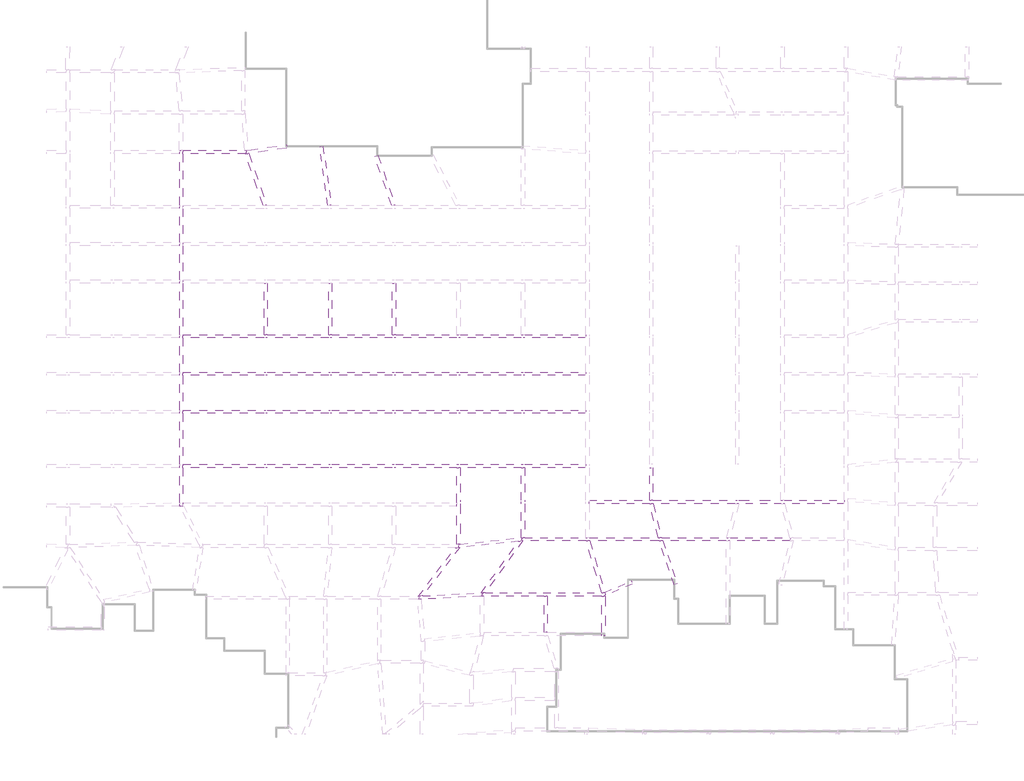
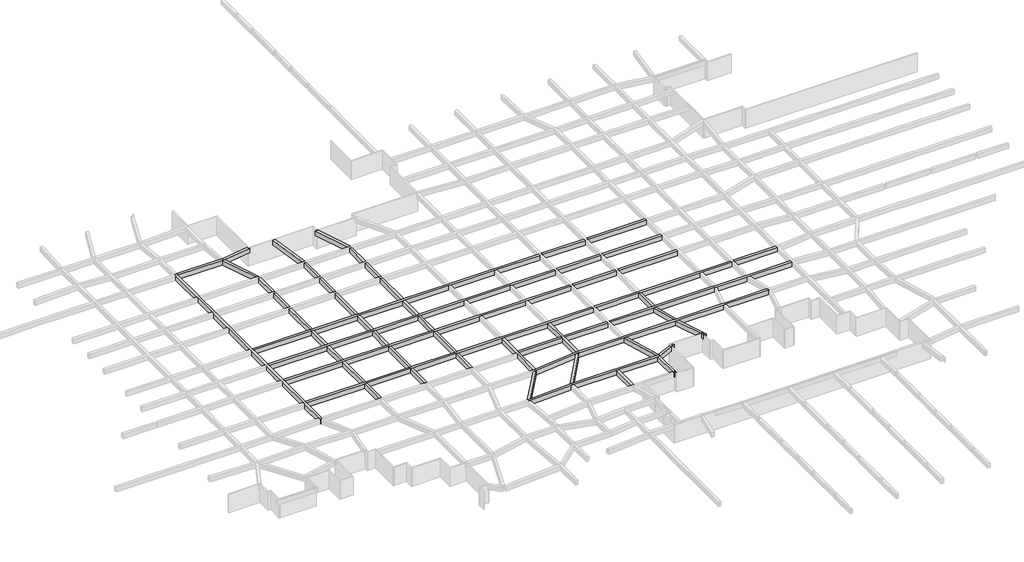
# One storey, part 33 of 45: 29 beams.
"""IFC4 building model written with IfcOpenShell, lengths in millimetres."""

from ifc_helpers import new_model, si_unit, frame, origin, place, context, project, spatial, polyline, outline, extrude, faceted_brep, element, save

model = new_model("IFC4")

# Units and contexts
model_context = context("Model", 3, world=origin())
ifc_project = project(units=[si_unit("LENGTHUNIT", "METRE", prefix="MILLI")], contexts=[model_context])

# Site, building, storey
site = spatial("IfcSite", under=ifc_project)
building = spatial("IfcBuilding", under=site)
storey = spatial("IfcBuildingStorey", under=building, Name="户型图", Elevation=0.0)

# Beams
placement = place(None, origin())
element("IfcBeam", 1, ObjectType="混凝土 - 矩形梁 : KL_beam", at=placement, inside=storey, context=model_context, shape_type="Brep", body=[
    faceted_brep([(-62329.0040152, 126289.9393475, 3300.0), (-62333.0898312, 126289.9393475, 3300.0), (-62729.0040152, 126289.9393475, 3300.0), (-62729.0040152, 125889.9393475, 3300.0), (-62729.0040152, 119677.6221749, 3300.0), (-62729.0040152, 119277.6221749, 3300.0), (-62729.0040152, 115171.853595, 3300.0), (-62729.0040152, 114771.853595, 3300.0), (-62729.0040152, 110629.932653, 3300.0), (-62729.0040152, 110229.932653, 3300.0), (-62729.0040152, 104011.2459144, 3300.0), (-62729.0040152, 103611.2459144, 3300.0), (-62729.0040152, 99488.7126183, 3300.0), (-62729.0040152, 99088.7126183, 3300.0), (-62729.0040152, 94888.7126183, 3300.0), (-62729.0040152, 94488.7126183, 3300.0), (-62729.0040152, 88347.4925836, 3300.0), (-62729.0040152, 87947.4925836, 3300.0), (-62729.0040152, 83686.8868717, 3300.0), (-62729.0040152, 83286.8331799, 3300.0), (-62652.5301432, 83288.0862256, 3300.0), (-62527.3655972, 83290.1370817, 3300.0), (-62329.0040152, 83293.3872917, 3300.0), (-62329.0040152, 83690.1370817, 3300.0), (-62329.0040152, 87947.4925836, 3300.0), (-62329.0040152, 88347.4925836, 3300.0), (-62329.0040152, 94488.7126183, 3300.0), (-62329.0040152, 94888.7126183, 3300.0), (-62329.0040152, 99088.7126183, 3300.0), (-62329.0040152, 99488.7126183, 3300.0), (-62329.0040152, 103611.2459144, 3300.0), (-62329.0040152, 104011.2459144, 3300.0), (-62329.0040152, 110229.932653, 3300.0), (-62329.0040152, 110629.932653, 3300.0), (-62329.0040152, 114771.853595, 3300.0), (-62329.0040152, 115171.853595, 3300.0), (-62329.0040152, 119262.5591329, 3300.0), (-62329.0040152, 119662.5591329, 3300.0), (-62329.0040152, 125890.334816, 3300.0), (-62729.0040152, 126289.9393475, 2500.0), (-62729.0040152, 125889.9393475, 2500.0), (-62729.0040152, 119677.6221749, 2500.0), (-62729.0040152, 119277.6221749, 2500.0), (-62729.0040152, 115171.853595, 2500.0), (-62729.0040152, 114771.853595, 2500.0), (-62729.0040152, 110629.932653, 2500.0), (-62729.0040152, 110229.932653, 2500.0), (-62729.0040152, 104011.2459144, 2500.0), (-62729.0040152, 103611.2459144, 2500.0), (-62729.0040152, 99488.7126183, 2500.0), (-62729.0040152, 99088.7126183, 2500.0), (-62729.0040152, 94888.7126183, 2500.0), (-62729.0040152, 94488.7126183, 2500.0), (-62729.0040152, 88347.4925836, 2500.0), (-62729.0040152, 87947.4925836, 2500.0), (-62729.0040152, 83686.8868717, 2500.0), (-62729.0040152, 83286.8331799, 2500.0), (-62333.0898312, 126289.9393475, 2500.0), (-62329.0040152, 126289.9393475, 2500.0), (-62329.0040152, 125890.334816, 2500.0), (-62329.0040152, 119662.5591329, 2500.0), (-62329.0040152, 119262.5591329, 2500.0), (-62329.0040152, 115171.853595, 2500.0), (-62329.0040152, 114771.853595, 2500.0), (-62329.0040152, 110629.932653, 2500.0), (-62329.0040152, 110229.932653, 2500.0), (-62329.0040152, 104011.2459144, 2500.0), (-62329.0040152, 103611.2459144, 2500.0), (-62329.0040152, 99488.7126183, 2500.0), (-62329.0040152, 99088.7126183, 2500.0), (-62329.0040152, 94888.7126183, 2500.0), (-62329.0040152, 94488.7126183, 2500.0), (-62329.0040152, 88347.4925836, 2500.0), (-62329.0040152, 87947.4925836, 2500.0), (-62329.0040152, 83690.1370817, 2500.0), (-62329.0040152, 83293.3872917, 2500.0), (-62527.3655972, 83290.1370817, 2500.0), (-62652.5301432, 83288.0862256, 2500.0)], [[[0, 1, 2, 3, 4, 5, 6, 7, 8, 9, 10, 11, 12, 13, 14, 15, 16, 17, 18, 19, 20, 21, 22, 23, 24, 25, 26, 27, 28, 29, 30, 31, 32, 33, 34, 35, 36, 37, 38]], [[2, 39, 40, 41, 42, 43, 44, 45, 46, 47, 48, 49, 50, 51, 52, 53, 54, 55, 56, 19, 18, 17, 16, 15, 14, 13, 12, 11, 10, 9, 8, 7, 6, 5, 4, 3]], [[39, 57, 58, 59, 60, 61, 62, 63, 64, 65, 66, 67, 68, 69, 70, 71, 72, 73, 74, 75, 76, 77, 56, 55, 54, 53, 52, 51, 50, 49, 48, 47, 46, 45, 44, 43, 42, 41, 40]], [[58, 0, 38, 37, 36, 35, 34, 33, 32, 31, 30, 29, 28, 27, 26, 25, 24, 23, 22, 75, 74, 73, 72, 71, 70, 69, 68, 67, 66, 65, 64, 63, 62, 61, 60, 59]], [[2, 1, 0, 58, 57, 39]], [[22, 21, 20, 19, 56, 77, 76, 75]]]),
])
element("IfcBeam", 2, ObjectType="混凝土 - 矩形梁 : KL_beam", at=placement, inside=storey, context=model_context, shape_type="Brep", body=[
    faceted_brep([(-62329.0040152, 125890.334816, 3300.0), (-54774.8544543, 125890.334816, 3300.0), (-54619.1044688, 125890.334816, 3300.0), (-54647.0751936, 126290.334816, 3300.0), (-54849.9735336, 126290.334816, 3300.0), (-62333.0898312, 126290.334816, 3300.0), (-62333.0898312, 126289.9393475, 3300.0), (-62329.0040152, 126289.9393475, 3300.0), (-62329.0040152, 125890.334816, 2500.0), (-54774.8544543, 125890.334816, 2500.0), (-54619.1044688, 125890.334816, 2500.0), (-62329.0040152, 126289.9393475, 2500.0), (-62333.0898312, 126289.9393475, 2500.0), (-62333.0898312, 126290.334816, 2500.0), (-54849.9735336, 126290.334816, 2500.0), (-54647.0751936, 126290.334816, 2500.0)], [[[0, 1, 2, 3, 4, 5, 6, 7]], [[2, 1, 0, 8, 9, 10]], [[10, 9, 8, 11, 12, 13, 14, 15]], [[3, 15, 14, 13, 5, 4]], [[7, 11, 8, 0]], [[11, 7, 6, 12]], [[6, 5, 13, 12]], [[3, 2, 10, 15]]]),
])
element("IfcBeam", 3, ObjectType="混凝土 - 矩形梁 : KL_beam", at=placement, inside=storey, context=model_context, shape_type="Brep", body=[
    faceted_brep([(-49808.6109146, 126970.3366244, 3300.0), (-49752.9416742, 126574.2293969, 3300.0), (-49752.9416742, 126574.2293969, 2500.0), (-49808.6109146, 126970.3366244, 2500.0), (-54450.8961138, 126317.9059876, 3300.0), (-54647.0751936, 126290.334816, 3300.0), (-54619.1044688, 125890.334816, 3300.0), (-54363.5430901, 125926.2516255, 3300.0), (-54619.1044688, 125890.334816, 2500.0), (-54363.5430901, 125926.2516255, 2500.0), (-54647.0751936, 126290.334816, 2500.0), (-54450.8961138, 126317.9059876, 2500.0)], [[[0, 1, 2, 3]], [[1, 0, 4, 5, 6, 7]], [[2, 1, 7, 6, 8, 9]], [[3, 2, 9, 8, 10, 11]], [[0, 3, 11, 10, 5, 4]], [[5, 10, 8, 6]]]),
])
element("IfcBeam", 4, ObjectType="混凝土 - 矩形梁 : KL_beam", at=placement, inside=storey, context=model_context, shape_type="Brep", body=[
    faceted_brep([(-62329.0040152, 104011.2459144, 3300.0), (-62329.0040152, 103611.2459144, 3300.0), (-52507.1090692, 103611.2459144, 3300.0), (-52107.1090692, 103611.2459144, 3300.0), (-44707.1090692, 103611.2459144, 3300.0), (-44307.1090692, 103611.2459144, 3300.0), (-36987.1090692, 103611.2459144, 3300.0), (-36587.1090692, 103611.2459144, 3300.0), (-29187.1090692, 103611.2459144, 3300.0), (-28787.1090692, 103611.2459144, 3300.0), (-21387.1090692, 103611.2459144, 3300.0), (-20987.1090692, 103611.2459144, 3300.0), (-13620.6748317, 103611.2459144, 3300.0), (-13620.6748317, 104011.2459144, 3300.0), (-20987.1090692, 104011.2459144, 3300.0), (-21387.1090692, 104011.2459144, 3300.0), (-28787.1090692, 104011.2459144, 3300.0), (-29187.1090692, 104011.2459144, 3300.0), (-36587.1090692, 104011.2459144, 3300.0), (-36987.1090692, 104011.2459144, 3300.0), (-44307.1090692, 104011.2459144, 3300.0), (-44707.1090692, 104011.2459144, 3300.0), (-52107.1090692, 104011.2459144, 3300.0), (-52507.1090692, 104011.2459144, 3300.0), (-62329.0040152, 103611.2459144, 2500.0), (-52507.1090692, 103611.2459144, 2500.0), (-52107.1090692, 103611.2459144, 2500.0), (-44707.1090692, 103611.2459144, 2500.0), (-44307.1090692, 103611.2459144, 2500.0), (-36987.1090692, 103611.2459144, 2500.0), (-36587.1090692, 103611.2459144, 2500.0), (-29187.1090692, 103611.2459144, 2500.0), (-28787.1090692, 103611.2459144, 2500.0), (-21387.1090692, 103611.2459144, 2500.0), (-20987.1090692, 103611.2459144, 2500.0), (-13620.6748317, 103611.2459144, 2500.0), (-62329.0040152, 104011.2459144, 2500.0), (-52507.1090692, 104011.2459144, 2500.0), (-52107.1090692, 104011.2459144, 2500.0), (-44707.1090692, 104011.2459144, 2500.0), (-44307.1090692, 104011.2459144, 2500.0), (-36987.1090692, 104011.2459144, 2500.0), (-36587.1090692, 104011.2459144, 2500.0), (-29187.1090692, 104011.2459144, 2500.0), (-28787.1090692, 104011.2459144, 2500.0), (-21387.1090692, 104011.2459144, 2500.0), (-20987.1090692, 104011.2459144, 2500.0), (-13620.6748317, 104011.2459144, 2500.0)], [[[0, 1, 2, 3, 4, 5, 6, 7, 8, 9, 10, 11, 12, 13, 14, 15, 16, 17, 18, 19, 20, 21, 22, 23]], [[1, 24, 25, 26, 27, 28, 29, 30, 31, 32, 33, 34, 35, 12, 11, 10, 9, 8, 7, 6, 5, 4, 3, 2]], [[24, 36, 37, 38, 39, 40, 41, 42, 43, 44, 45, 46, 47, 35, 34, 33, 32, 31, 30, 29, 28, 27, 26, 25]], [[36, 0, 23, 22, 21, 20, 19, 18, 17, 16, 15, 14, 13, 47, 46, 45, 44, 43, 42, 41, 40, 39, 38, 37]], [[1, 0, 36, 24]], [[13, 12, 35, 47]]]),
    faceted_brep([(-13220.6748317, 103611.2459144, 3300.0), (-13220.6748317, 104011.2459144, 3300.0), (-13220.6748317, 104011.2459144, 2500.0), (-13220.6748317, 103611.2459144, 2500.0), (-5904.3123934, 104011.2459144, 3300.0), (-5904.3123934, 103611.2459144, 3300.0), (-5904.3123934, 103611.2459144, 2500.0), (-5904.3123934, 104011.2459144, 2500.0)], [[[0, 1, 2, 3]], [[4, 5, 6, 7]], [[1, 0, 5, 4]], [[0, 3, 6, 5]], [[3, 2, 7, 6]], [[2, 1, 4, 7]]]),
    faceted_brep([(-5504.3123934, 104011.2459144, 3300.0), (-5504.3123934, 103611.2459144, 3300.0), (4500.9990644, 103611.2459144, 3300.0), (4500.9990644, 104011.2459144, 3300.0), (-5504.3123934, 103611.2459144, 2500.0), (4500.9990644, 103611.2459144, 2500.0), (-5504.3123934, 104011.2459144, 2500.0), (4500.9990644, 104011.2459144, 2500.0)], [[[0, 1, 2, 3]], [[1, 4, 5, 2]], [[4, 6, 7, 5]], [[6, 0, 3, 7]], [[1, 0, 6, 4]], [[3, 2, 5, 7]]]),
])
element("IfcBeam", 5, ObjectType="混凝土 - 矩形梁 : KL_beam", at=placement, inside=storey, context=model_context, shape_type="Brep", body=[
    faceted_brep([(-62329.0040152, 99488.7126183, 3300.0), (-62329.0040152, 99088.7126183, 3300.0), (-52507.1090692, 99088.7126183, 3300.0), (-52107.1090692, 99088.7126183, 3300.0), (-44707.1090692, 99088.7126183, 3300.0), (-44307.1090692, 99088.7126183, 3300.0), (-36987.1090692, 99088.7126183, 3300.0), (-36587.1090692, 99088.7126183, 3300.0), (-29187.1090692, 99088.7126183, 3300.0), (-28787.1090692, 99088.7126183, 3300.0), (-21387.1090692, 99088.7126183, 3300.0), (-20987.1090692, 99088.7126183, 3300.0), (-13620.6748317, 99088.7126183, 3300.0), (-13620.6748317, 99488.7126183, 3300.0), (-20987.1090692, 99488.7126183, 3300.0), (-21387.1090692, 99488.7126183, 3300.0), (-28787.1090692, 99488.7126183, 3300.0), (-29187.1090692, 99488.7126183, 3300.0), (-36587.1090692, 99488.7126183, 3300.0), (-36987.1090692, 99488.7126183, 3300.0), (-44307.1090692, 99488.7126183, 3300.0), (-44707.1090692, 99488.7126183, 3300.0), (-52107.1090692, 99488.7126183, 3300.0), (-52507.1090692, 99488.7126183, 3300.0), (-62329.0040152, 99088.7126183, 2500.0), (-52507.1090692, 99088.7126183, 2500.0), (-52107.1090692, 99088.7126183, 2500.0), (-44707.1090692, 99088.7126183, 2500.0), (-44307.1090692, 99088.7126183, 2500.0), (-36987.1090692, 99088.7126183, 2500.0), (-36587.1090692, 99088.7126183, 2500.0), (-29187.1090692, 99088.7126183, 2500.0), (-28787.1090692, 99088.7126183, 2500.0), (-21387.1090692, 99088.7126183, 2500.0), (-20987.1090692, 99088.7126183, 2500.0), (-13620.6748317, 99088.7126183, 2500.0), (-62329.0040152, 99488.7126183, 2500.0), (-52507.1090692, 99488.7126183, 2500.0), (-52107.1090692, 99488.7126183, 2500.0), (-44707.1090692, 99488.7126183, 2500.0), (-44307.1090692, 99488.7126183, 2500.0), (-36987.1090692, 99488.7126183, 2500.0), (-36587.1090692, 99488.7126183, 2500.0), (-29187.1090692, 99488.7126183, 2500.0), (-28787.1090692, 99488.7126183, 2500.0), (-21387.1090692, 99488.7126183, 2500.0), (-20987.1090692, 99488.7126183, 2500.0), (-13620.6748317, 99488.7126183, 2500.0)], [[[0, 1, 2, 3, 4, 5, 6, 7, 8, 9, 10, 11, 12, 13, 14, 15, 16, 17, 18, 19, 20, 21, 22, 23]], [[1, 24, 25, 26, 27, 28, 29, 30, 31, 32, 33, 34, 35, 12, 11, 10, 9, 8, 7, 6, 5, 4, 3, 2]], [[24, 36, 37, 38, 39, 40, 41, 42, 43, 44, 45, 46, 47, 35, 34, 33, 32, 31, 30, 29, 28, 27, 26, 25]], [[36, 0, 23, 22, 21, 20, 19, 18, 17, 16, 15, 14, 13, 47, 46, 45, 44, 43, 42, 41, 40, 39, 38, 37]], [[1, 0, 36, 24]], [[13, 12, 35, 47]]]),
    faceted_brep([(-13220.6748317, 99088.7126183, 3300.0), (-13220.6748317, 99488.7126183, 3300.0), (-13220.6748317, 99488.7126183, 2500.0), (-13220.6748317, 99088.7126183, 2500.0), (-5904.3123934, 99488.7126183, 3300.0), (-5904.3123934, 99088.7126183, 3300.0), (-5904.3123934, 99088.7126183, 2500.0), (-5904.3123934, 99488.7126183, 2500.0)], [[[0, 1, 2, 3]], [[4, 5, 6, 7]], [[1, 0, 5, 4]], [[0, 3, 6, 5]], [[3, 2, 7, 6]], [[2, 1, 4, 7]]]),
    faceted_brep([(-5504.3123934, 99488.7126183, 3300.0), (-5504.3123934, 99088.7126183, 3300.0), (4500.9990644, 99088.7126183, 3300.0), (4500.9990644, 99488.7126183, 3300.0), (-5504.3123934, 99088.7126183, 2500.0), (4500.9990644, 99088.7126183, 2500.0), (-5504.3123934, 99488.7126183, 2500.0), (4500.9990644, 99488.7126183, 2500.0)], [[[0, 1, 2, 3]], [[1, 4, 5, 2]], [[4, 6, 7, 5]], [[6, 0, 3, 7]], [[1, 0, 6, 4]], [[3, 2, 5, 7]]]),
])
element("IfcBeam", 6, ObjectType="混凝土 - 矩形梁 : KL_beam", at=placement, inside=storey, context=model_context, shape_type="Brep", body=[
    faceted_brep([(-62329.0040152, 94888.7126183, 3300.0), (-62329.0040152, 94488.7126183, 3300.0), (-52507.1090692, 94488.7126183, 3300.0), (-52107.1090692, 94488.7126183, 3300.0), (-44707.1090692, 94488.7126183, 3300.0), (-44307.1090692, 94488.7126183, 3300.0), (-36987.1090692, 94488.7126183, 3300.0), (-36587.1090692, 94488.7126183, 3300.0), (-29187.1090692, 94488.7126183, 3300.0), (-28787.1090692, 94488.7126183, 3300.0), (-21387.1090692, 94488.7126183, 3300.0), (-20987.1090692, 94488.7126183, 3300.0), (-13620.6748317, 94488.7126183, 3300.0), (-13620.6748317, 94888.7126183, 3300.0), (-20987.1090692, 94888.7126183, 3300.0), (-21387.1090692, 94888.7126183, 3300.0), (-28787.1090692, 94888.7126183, 3300.0), (-29187.1090692, 94888.7126183, 3300.0), (-36587.1090692, 94888.7126183, 3300.0), (-36987.1090692, 94888.7126183, 3300.0), (-44307.1090692, 94888.7126183, 3300.0), (-44707.1090692, 94888.7126183, 3300.0), (-52107.1090692, 94888.7126183, 3300.0), (-52507.1090692, 94888.7126183, 3300.0), (-62329.0040152, 94488.7126183, 2500.0), (-52507.1090692, 94488.7126183, 2500.0), (-52107.1090692, 94488.7126183, 2500.0), (-44707.1090692, 94488.7126183, 2500.0), (-44307.1090692, 94488.7126183, 2500.0), (-36987.1090692, 94488.7126183, 2500.0), (-36587.1090692, 94488.7126183, 2500.0), (-29187.1090692, 94488.7126183, 2500.0), (-28787.1090692, 94488.7126183, 2500.0), (-21387.1090692, 94488.7126183, 2500.0), (-20987.1090692, 94488.7126183, 2500.0), (-13620.6748317, 94488.7126183, 2500.0), (-62329.0040152, 94888.7126183, 2500.0), (-52507.1090692, 94888.7126183, 2500.0), (-52107.1090692, 94888.7126183, 2500.0), (-44707.1090692, 94888.7126183, 2500.0), (-44307.1090692, 94888.7126183, 2500.0), (-36987.1090692, 94888.7126183, 2500.0), (-36587.1090692, 94888.7126183, 2500.0), (-29187.1090692, 94888.7126183, 2500.0), (-28787.1090692, 94888.7126183, 2500.0), (-21387.1090692, 94888.7126183, 2500.0), (-20987.1090692, 94888.7126183, 2500.0), (-13620.6748317, 94888.7126183, 2500.0)], [[[0, 1, 2, 3, 4, 5, 6, 7, 8, 9, 10, 11, 12, 13, 14, 15, 16, 17, 18, 19, 20, 21, 22, 23]], [[1, 24, 25, 26, 27, 28, 29, 30, 31, 32, 33, 34, 35, 12, 11, 10, 9, 8, 7, 6, 5, 4, 3, 2]], [[24, 36, 37, 38, 39, 40, 41, 42, 43, 44, 45, 46, 47, 35, 34, 33, 32, 31, 30, 29, 28, 27, 26, 25]], [[36, 0, 23, 22, 21, 20, 19, 18, 17, 16, 15, 14, 13, 47, 46, 45, 44, 43, 42, 41, 40, 39, 38, 37]], [[1, 0, 36, 24]], [[13, 12, 35, 47]]]),
    faceted_brep([(-13220.6748317, 94488.7126183, 3300.0), (-13220.6748317, 94888.7126183, 3300.0), (-13220.6748317, 94888.7126183, 2500.0), (-13220.6748317, 94488.7126183, 2500.0), (-5904.3123934, 94888.7126183, 3300.0), (-5904.3123934, 94488.7126183, 3300.0), (-5904.3123934, 94488.7126183, 2500.0), (-5904.3123934, 94888.7126183, 2500.0)], [[[0, 1, 2, 3]], [[4, 5, 6, 7]], [[1, 0, 5, 4]], [[0, 3, 6, 5]], [[3, 2, 7, 6]], [[2, 1, 4, 7]]]),
    faceted_brep([(-5504.3123934, 94888.7126183, 3300.0), (-5504.3123934, 94488.7126183, 3300.0), (4500.9990644, 94488.7126183, 3300.0), (4500.9990644, 94888.7126183, 3300.0), (-5504.3123934, 94488.7126183, 2500.0), (4500.9990644, 94488.7126183, 2500.0), (-5504.3123934, 94888.7126183, 2500.0), (4500.9990644, 94888.7126183, 2500.0)], [[[0, 1, 2, 3]], [[1, 4, 5, 2]], [[4, 6, 7, 5]], [[6, 0, 3, 7]], [[1, 0, 6, 4]], [[3, 2, 5, 7]]]),
])
element("IfcBeam", 7, ObjectType="混凝土 - 矩形梁 : KL_beam", at=placement, inside=storey, context=model_context, shape_type="Brep", body=[
    faceted_brep([(-62329.0040152, 88347.4925836, 3300.0), (-62329.0040152, 87947.4925836, 3300.0), (-52507.1090692, 87947.4925836, 3300.0), (-52107.1090692, 87947.4925836, 3300.0), (-44707.1090692, 87947.4925836, 3300.0), (-44307.1090692, 87947.4925836, 3300.0), (-36987.1090692, 87947.4925836, 3300.0), (-36587.1090692, 87947.4925836, 3300.0), (-29187.1090692, 87947.4925836, 3300.0), (-28787.1090692, 87947.4925836, 3300.0), (-21387.1090692, 87947.4925836, 3300.0), (-20987.1090692, 87947.4925836, 3300.0), (-13620.6748317, 87947.4925836, 3300.0), (-13620.6748317, 88347.4925836, 3300.0), (-20987.1090692, 88347.4925836, 3300.0), (-21387.1090692, 88347.4925836, 3300.0), (-28787.1090692, 88347.4925836, 3300.0), (-29187.1090692, 88347.4925836, 3300.0), (-36587.1090692, 88347.4925836, 3300.0), (-36987.1090692, 88347.4925836, 3300.0), (-44307.1090692, 88347.4925836, 3300.0), (-44707.1090692, 88347.4925836, 3300.0), (-52107.1090692, 88347.4925836, 3300.0), (-52507.1090692, 88347.4925836, 3300.0), (-62329.0040152, 87947.4925836, 2500.0), (-52507.1090692, 87947.4925836, 2500.0), (-52107.1090692, 87947.4925836, 2500.0), (-44707.1090692, 87947.4925836, 2500.0), (-44307.1090692, 87947.4925836, 2500.0), (-36987.1090692, 87947.4925836, 2500.0), (-36587.1090692, 87947.4925836, 2500.0), (-29187.1090692, 87947.4925836, 2500.0), (-28787.1090692, 87947.4925836, 2500.0), (-21387.1090692, 87947.4925836, 2500.0), (-20987.1090692, 87947.4925836, 2500.0), (-13620.6748317, 87947.4925836, 2500.0), (-62329.0040152, 88347.4925836, 2500.0), (-52507.1090692, 88347.4925836, 2500.0), (-52107.1090692, 88347.4925836, 2500.0), (-44707.1090692, 88347.4925836, 2500.0), (-44307.1090692, 88347.4925836, 2500.0), (-36987.1090692, 88347.4925836, 2500.0), (-36587.1090692, 88347.4925836, 2500.0), (-29187.1090692, 88347.4925836, 2500.0), (-28787.1090692, 88347.4925836, 2500.0), (-21387.1090692, 88347.4925836, 2500.0), (-20987.1090692, 88347.4925836, 2500.0), (-13620.6748317, 88347.4925836, 2500.0)], [[[0, 1, 2, 3, 4, 5, 6, 7, 8, 9, 10, 11, 12, 13, 14, 15, 16, 17, 18, 19, 20, 21, 22, 23]], [[1, 24, 25, 26, 27, 28, 29, 30, 31, 32, 33, 34, 35, 12, 11, 10, 9, 8, 7, 6, 5, 4, 3, 2]], [[24, 36, 37, 38, 39, 40, 41, 42, 43, 44, 45, 46, 47, 35, 34, 33, 32, 31, 30, 29, 28, 27, 26, 25]], [[36, 0, 23, 22, 21, 20, 19, 18, 17, 16, 15, 14, 13, 47, 46, 45, 44, 43, 42, 41, 40, 39, 38, 37]], [[1, 0, 36, 24]], [[13, 12, 35, 47]]]),
    faceted_brep([(17658.0309094, 88347.4925836, 3300.0), (17658.0309094, 87947.4925836, 3300.0), (17658.0309094, 87947.4925836, 2500.0), (17658.0309094, 88347.4925836, 2500.0), (10373.3027926, 87947.4925836, 3300.0), (10373.3027926, 88347.4925836, 3300.0), (10373.3027926, 88347.4925836, 2500.0), (10373.3027926, 87947.4925836, 2500.0)], [[[0, 1, 2, 3]], [[4, 5, 6, 7]], [[1, 0, 5, 4]], [[2, 1, 4, 7]], [[3, 2, 7, 6]], [[0, 3, 6, 5]]]),
    faceted_brep([(9973.3027926, 88347.4925836, 3300.0), (9973.3027926, 87947.4925836, 3300.0), (9973.3027926, 87947.4925836, 2500.0), (9973.3027926, 88347.4925836, 2500.0), (-13220.6748317, 87947.4925836, 3300.0), (-13220.6748317, 88347.4925836, 3300.0), (-13220.6748317, 88347.4925836, 2500.0), (-13220.6748317, 87947.4925836, 2500.0), (4900.9990644, 88347.4925836, 3300.0), (4500.9990644, 88347.4925836, 3300.0), (-5504.3123934, 88347.4925836, 3300.0), (-5904.3123934, 88347.4925836, 3300.0), (-5904.3123934, 87947.4925836, 3300.0), (-5504.3123934, 87947.4925836, 3300.0), (4500.9990644, 87947.4925836, 3300.0), (4900.9990644, 87947.4925836, 3300.0), (-5904.3123934, 87947.4925836, 2500.0), (-5504.3123934, 87947.4925836, 2500.0), (4500.9990644, 87947.4925836, 2500.0), (4900.9990644, 87947.4925836, 2500.0), (-5904.3123934, 88347.4925836, 2500.0), (-5504.3123934, 88347.4925836, 2500.0), (4500.9990644, 88347.4925836, 2500.0), (4900.9990644, 88347.4925836, 2500.0)], [[[0, 1, 2, 3]], [[4, 5, 6, 7]], [[1, 0, 8, 9, 10, 11, 5, 4, 12, 13, 14, 15]], [[2, 1, 15, 14, 13, 12, 4, 7, 16, 17, 18, 19]], [[3, 2, 19, 18, 17, 16, 7, 6, 20, 21, 22, 23]], [[0, 3, 23, 22, 21, 20, 6, 5, 11, 10, 9, 8]]]),
])
element("IfcBeam", 8, ObjectType="混凝土 - 矩形梁 : KL_beam", at=placement, inside=storey, context=model_context, shape_type="SweptSolid", body=[
    extrude(outline(polyline([(-5904.3123934, 87947.4925836), (-5504.3123934, 87947.4925836), (-5504.3123934, 83990.1370817), (-5904.3123934, 83990.1370817), (-5904.3123934, 87947.4925836)])), frame((0.0, 0.0, 2500.0), z_axis=(0.0, 0.0, 1.0), x_axis=(1.0, 0.0, 0.0)), (0.0, 0.0, 1.0), 800.0),
])
element("IfcBeam", 9, ObjectType="混凝土 - 矩形梁 : KL_beam", at=placement, inside=storey, context=model_context, shape_type="SweptSolid", body=[
    extrude(outline(polyline([(-36587.1090692, 83690.1370817), (-36987.1090692, 83690.1370817), (-36987.1090692, 87947.4925836), (-36587.1090692, 87947.4925836), (-36587.1090692, 83690.1370817)])), frame((0.0, 0.0, 2500.0), z_axis=(0.0, 0.0, 1.0), x_axis=(1.0, 0.0, 0.0)), (0.0, 0.0, 1.0), 800.0),
    extrude(outline(polyline([(-36987.1090692, 119262.5591329), (-36587.1090692, 119262.5591329), (-36587.1090692, 115171.853595), (-36987.1090692, 115171.853595), (-36987.1090692, 119262.5591329)])), frame((0.0, 0.0, 2500.0), z_axis=(0.0, 0.0, 1.0), x_axis=(1.0, 0.0, 0.0)), (0.0, 0.0, 1.0), 800.0),
    extrude(outline(polyline([(-36987.1090692, 114771.853595), (-36587.1090692, 114771.853595), (-36587.1090692, 110629.932653), (-36987.1090692, 110629.932653), (-36987.1090692, 114771.853595)])), frame((0.0, 0.0, 2500.0), z_axis=(0.0, 0.0, 1.0), x_axis=(1.0, 0.0, 0.0)), (0.0, 0.0, 1.0), 800.0),
    extrude(outline(polyline([(-36987.1090692, 110229.932653), (-36587.1090692, 110229.932653), (-36587.1090692, 104011.2459144), (-36987.1090692, 104011.2459144), (-36987.1090692, 110229.932653)])), frame((0.0, 0.0, 2500.0), z_axis=(0.0, 0.0, 1.0), x_axis=(1.0, 0.0, 0.0)), (0.0, 0.0, 1.0), 800.0),
    extrude(outline(polyline([(-36987.1090692, 103611.2459144), (-36587.1090692, 103611.2459144), (-36587.1090692, 99488.7126183), (-36987.1090692, 99488.7126183), (-36987.1090692, 103611.2459144)])), frame((0.0, 0.0, 2500.0), z_axis=(0.0, 0.0, 1.0), x_axis=(1.0, 0.0, 0.0)), (0.0, 0.0, 1.0), 800.0),
    extrude(outline(polyline([(-36987.1090692, 99088.7126183), (-36587.1090692, 99088.7126183), (-36587.1090692, 94888.7126183), (-36987.1090692, 94888.7126183), (-36987.1090692, 99088.7126183)])), frame((0.0, 0.0, 2500.0), z_axis=(0.0, 0.0, 1.0), x_axis=(1.0, 0.0, 0.0)), (0.0, 0.0, 1.0), 800.0),
    extrude(outline(polyline([(-36987.1090692, 94488.7126183), (-36587.1090692, 94488.7126183), (-36587.1090692, 88347.4925836), (-36987.1090692, 88347.4925836), (-36987.1090692, 94488.7126183)])), frame((0.0, 0.0, 2500.0), z_axis=(0.0, 0.0, 1.0), x_axis=(1.0, 0.0, 0.0)), (0.0, 0.0, 1.0), 800.0),
])
element("IfcBeam", 10, ObjectType="混凝土 - 矩形梁 : KL_beam", at=placement, inside=storey, context=model_context, shape_type="SweptSolid", body=[
    extrude(outline(polyline([(-44707.1090692, 119262.5591329), (-44307.1090692, 119262.5591329), (-44307.1090692, 115171.853595), (-44707.1090692, 115171.853595), (-44707.1090692, 119262.5591329)])), frame((0.0, 0.0, 2500.0), z_axis=(0.0, 0.0, 1.0), x_axis=(1.0, 0.0, 0.0)), (0.0, 0.0, 1.0), 800.0),
    extrude(outline(polyline([(-44307.1090692, 83690.1370817), (-44707.1090692, 83690.1370817), (-44707.1090692, 87947.4925836), (-44307.1090692, 87947.4925836), (-44307.1090692, 83690.1370817)])), frame((0.0, 0.0, 2500.0), z_axis=(0.0, 0.0, 1.0), x_axis=(1.0, 0.0, 0.0)), (0.0, 0.0, 1.0), 800.0),
    extrude(outline(polyline([(-44707.1090692, 114771.853595), (-44307.1090692, 114771.853595), (-44307.1090692, 110629.932653), (-44707.1090692, 110629.932653), (-44707.1090692, 114771.853595)])), frame((0.0, 0.0, 2500.0), z_axis=(0.0, 0.0, 1.0), x_axis=(1.0, 0.0, 0.0)), (0.0, 0.0, 1.0), 800.0),
    extrude(outline(polyline([(-44707.1090692, 110229.932653), (-44307.1090692, 110229.932653), (-44307.1090692, 104011.2459144), (-44707.1090692, 104011.2459144), (-44707.1090692, 110229.932653)])), frame((0.0, 0.0, 2500.0), z_axis=(0.0, 0.0, 1.0), x_axis=(1.0, 0.0, 0.0)), (0.0, 0.0, 1.0), 800.0),
    extrude(outline(polyline([(-44707.1090692, 103611.2459144), (-44307.1090692, 103611.2459144), (-44307.1090692, 99488.7126183), (-44707.1090692, 99488.7126183), (-44707.1090692, 103611.2459144)])), frame((0.0, 0.0, 2500.0), z_axis=(0.0, 0.0, 1.0), x_axis=(1.0, 0.0, 0.0)), (0.0, 0.0, 1.0), 800.0),
    extrude(outline(polyline([(-44707.1090692, 99088.7126183), (-44307.1090692, 99088.7126183), (-44307.1090692, 94888.7126183), (-44707.1090692, 94888.7126183), (-44707.1090692, 99088.7126183)])), frame((0.0, 0.0, 2500.0), z_axis=(0.0, 0.0, 1.0), x_axis=(1.0, 0.0, 0.0)), (0.0, 0.0, 1.0), 800.0),
    extrude(outline(polyline([(-44707.1090692, 94488.7126183), (-44307.1090692, 94488.7126183), (-44307.1090692, 88347.4925836), (-44707.1090692, 88347.4925836), (-44707.1090692, 94488.7126183)])), frame((0.0, 0.0, 2500.0), z_axis=(0.0, 0.0, 1.0), x_axis=(1.0, 0.0, 0.0)), (0.0, 0.0, 1.0), 800.0),
])
element("IfcBeam", 11, ObjectType="混凝土 - 矩形梁 : KL_beam", at=placement, inside=storey, context=model_context, shape_type="SweptSolid", body=[
    extrude(outline(polyline([(-52107.1090692, 83690.1370817), (-52507.1090692, 83690.1370817), (-52507.1090692, 87947.4925836), (-52107.1090692, 87947.4925836), (-52107.1090692, 83690.1370817)])), frame((0.0, 0.0, 2500.0), z_axis=(0.0, 0.0, 1.0), x_axis=(1.0, 0.0, 0.0)), (0.0, 0.0, 1.0), 800.0),
    extrude(outline(polyline([(-52507.1090692, 119262.5591329), (-52107.1090692, 119262.5591329), (-52107.1090692, 115171.853595), (-52507.1090692, 115171.853595), (-52507.1090692, 119262.5591329)])), frame((0.0, 0.0, 2500.0), z_axis=(0.0, 0.0, 1.0), x_axis=(1.0, 0.0, 0.0)), (0.0, 0.0, 1.0), 800.0),
    extrude(outline(polyline([(-52507.1090692, 114771.853595), (-52107.1090692, 114771.853595), (-52107.1090692, 110629.932653), (-52507.1090692, 110629.932653), (-52507.1090692, 114771.853595)])), frame((0.0, 0.0, 2500.0), z_axis=(0.0, 0.0, 1.0), x_axis=(1.0, 0.0, 0.0)), (0.0, 0.0, 1.0), 800.0),
    extrude(outline(polyline([(-52507.1090692, 110229.932653), (-52107.1090692, 110229.932653), (-52107.1090692, 104011.2459144), (-52507.1090692, 104011.2459144), (-52507.1090692, 110229.932653)])), frame((0.0, 0.0, 2500.0), z_axis=(0.0, 0.0, 1.0), x_axis=(1.0, 0.0, 0.0)), (0.0, 0.0, 1.0), 800.0),
    extrude(outline(polyline([(-52507.1090692, 103611.2459144), (-52107.1090692, 103611.2459144), (-52107.1090692, 99488.7126183), (-52507.1090692, 99488.7126183), (-52507.1090692, 103611.2459144)])), frame((0.0, 0.0, 2500.0), z_axis=(0.0, 0.0, 1.0), x_axis=(1.0, 0.0, 0.0)), (0.0, 0.0, 1.0), 800.0),
    extrude(outline(polyline([(-52507.1090692, 99088.7126183), (-52107.1090692, 99088.7126183), (-52107.1090692, 94888.7126183), (-52507.1090692, 94888.7126183), (-52507.1090692, 99088.7126183)])), frame((0.0, 0.0, 2500.0), z_axis=(0.0, 0.0, 1.0), x_axis=(1.0, 0.0, 0.0)), (0.0, 0.0, 1.0), 800.0),
    extrude(outline(polyline([(-52507.1090692, 94488.7126183), (-52107.1090692, 94488.7126183), (-52107.1090692, 88347.4925836), (-52507.1090692, 88347.4925836), (-52507.1090692, 94488.7126183)])), frame((0.0, 0.0, 2500.0), z_axis=(0.0, 0.0, 1.0), x_axis=(1.0, 0.0, 0.0)), (0.0, 0.0, 1.0), 800.0),
])
element("IfcBeam", 12, ObjectType="混凝土 - 矩形梁 : KL_beam", at=placement, inside=storey, context=model_context, shape_type="SweptSolid", body=[
    extrude(outline(polyline([(-52165.4117003, 119662.5591329), (-52589.3274296, 119662.5591329), (-54774.8544543, 125890.334816), (-54619.1044688, 125890.334816), (-54363.5430901, 125926.2516255), (-52165.4117003, 119662.5591329)])), frame((0.0, 0.0, 2500.0), z_axis=(0.0, 0.0, 1.0), x_axis=(1.0, 0.0, 0.0)), (0.0, 0.0, 1.0), 800.0),
])
element("IfcBeam", 13, ObjectType="混凝土 - 矩形梁 : KL_beam", at=placement, inside=storey, context=model_context, shape_type="SweptSolid", body=[
    extrude(outline(polyline([(-45785.1524788, 126735.0533212), (-45389.0452513, 126790.7225616), (-44387.2472132, 119662.5591329), (-44791.1782422, 119662.5591329), (-45785.1524788, 126735.0533212)])), frame((0.0, 0.0, 2500.0), z_axis=(0.0, 0.0, 1.0), x_axis=(1.0, 0.0, 0.0)), (0.0, 0.0, 1.0), 800.0),
])
element("IfcBeam", 14, ObjectType="混凝土 - 矩形梁 : KL_beam", at=placement, inside=storey, context=model_context, shape_type="SweptSolid", body=[
    extrude(outline(polyline([(-39151.7265961, 125596.6775158), (-38774.29309, 125729.1310866), (-36645.3376446, 119662.5591329), (-37069.2533739, 119662.5591329), (-39151.7265961, 125596.6775158)])), frame((0.0, 0.0, 2500.0), z_axis=(0.0, 0.0, 1.0), x_axis=(1.0, 0.0, 0.0)), (0.0, 0.0, 1.0), 800.0),
])
element("IfcBeam", 15, ObjectType="混凝土 - 矩形梁 : KL_beam", at=placement, inside=storey, context=model_context, shape_type="Brep", body=[
    faceted_brep([(-21340.1829395, 79472.5341829, 3300.0), (-21319.2198278, 79072.5341829, 3300.0), (-21227.6444043, 79072.5341829, 3300.0), (-13569.5434013, 79072.5341829, 3300.0), (-13151.981446, 79072.5341829, 3300.0), (-4755.7287429, 79072.5341829, 3300.0), (-4332.2504281, 79072.5341829, 3300.0), (3388.0001812, 79072.5341829, 3300.0), (3788.0001812, 79072.5341829, 3300.0), (11052.0342818, 79072.5341829, 3300.0), (11151.7571818, 79072.5341829, 3300.0), (11052.0259807, 79472.5341829, 3300.0), (3843.9885077, 79472.5341829, 3300.0), (3431.7430559, 79472.5341829, 3300.0), (-4457.2556275, 79472.5341829, 3300.0), (-4869.5010792, 79472.5341829, 3300.0), (-13220.6748317, 79472.5341829, 3300.0), (-13620.6748317, 79472.5341829, 3300.0), (-20987.1090692, 79472.5341829, 3300.0), (-21340.1829395, 79472.5341829, 2500.0), (11052.0259807, 79472.5341829, 2500.0), (3843.9885077, 79472.5341829, 2500.0), (3431.7430559, 79472.5341829, 2500.0), (-4457.2556275, 79472.5341829, 2500.0), (-4869.5010792, 79472.5341829, 2500.0), (-13220.6748317, 79472.5341829, 2500.0), (-13620.6748317, 79472.5341829, 2500.0), (-20987.1090692, 79472.5341829, 2500.0), (-21319.2198278, 79072.5341829, 2500.0), (11151.7571818, 79072.5341829, 2500.0), (11052.0342818, 79072.5341829, 2500.0), (3788.0001812, 79072.5341829, 2500.0), (3388.0001812, 79072.5341829, 2500.0), (-4332.2504281, 79072.5341829, 2500.0), (-4755.7287429, 79072.5341829, 2500.0), (-13151.981446, 79072.5341829, 2500.0), (-13569.5434013, 79072.5341829, 2500.0), (-21227.6444043, 79072.5341829, 2500.0)], [[[0, 1, 2, 3, 4, 5, 6, 7, 8, 9, 10, 11, 12, 13, 14, 15, 16, 17, 18]], [[19, 0, 18, 17, 16, 15, 14, 13, 12, 11, 20, 21, 22, 23, 24, 25, 26, 27]], [[28, 19, 27, 26, 25, 24, 23, 22, 21, 20, 29, 30, 31, 32, 33, 34, 35, 36, 37]], [[1, 28, 37, 36, 35, 34, 33, 32, 31, 30, 29, 10, 9, 8, 7, 6, 5, 4, 3, 2]], [[1, 0, 19, 28]], [[11, 10, 29, 20]]]),
])
element("IfcBeam", 16, ObjectType="混凝土 - 矩形梁 : KL_beam", at=placement, inside=storey, context=model_context, shape_type="Brep", body=[
    faceted_brep([(-28977.0384221, 78267.6650157, 3300.0), (-28880.9990982, 78277.7591554, 3300.0), (-21754.8185448, 79026.7509129, 3300.0), (-21319.2198278, 79072.5341829, 3300.0), (-21340.1829395, 79472.5341829, 3300.0), (-21387.1090692, 79467.6020479, 3300.0), (-28787.1090692, 78689.830707, 3300.0), (-28998.0015338, 78667.6650157, 3300.0), (-21340.1829395, 79472.5341829, 2500.0), (-21387.1090692, 79467.6020479, 2500.0), (-28787.1090692, 78689.830707, 2500.0), (-28998.0015338, 78667.6650157, 2500.0), (-21319.2198278, 79072.5341829, 2500.0), (-21754.8185448, 79026.7509129, 2500.0), (-28880.9990982, 78277.7591554, 2500.0), (-28977.0384221, 78267.6650157, 2500.0)], [[[0, 1, 2, 3, 4, 5, 6, 7]], [[7, 6, 5, 4, 8, 9, 10, 11]], [[11, 10, 9, 8, 12, 13, 14, 15]], [[3, 2, 1, 0, 15, 14, 13, 12]], [[3, 12, 8, 4]], [[0, 7, 11, 15]]]),
])
element("IfcBeam", 17, ObjectType="混凝土 - 矩形梁 : KL_beam", at=placement, inside=storey, context=model_context, shape_type="Brep", body=[
    faceted_brep([(-28787.1090692, 87947.4925836, 3300.0), (-29187.1090692, 87947.4925836, 3300.0), (-29187.1090692, 83690.1370817, 3300.0), (-29187.1090692, 83290.1370817, 3300.0), (-29187.1090692, 78667.6650157, 3300.0), (-28998.0015338, 78667.6650157, 3300.0), (-28787.1090692, 78689.830707, 3300.0), (-28787.1090692, 83590.1370817, 3300.0), (-28787.1090692, 83990.1370817, 3300.0), (-29187.1090692, 87947.4925836, 2500.0), (-29187.1090692, 83690.1370817, 2500.0), (-29187.1090692, 83290.1370817, 2500.0), (-29187.1090692, 78667.6650157, 2500.0), (-28787.1090692, 87947.4925836, 2500.0), (-28787.1090692, 83990.1370817, 2500.0), (-28787.1090692, 83590.1370817, 2500.0), (-28787.1090692, 78689.830707, 2500.0), (-28998.0015338, 78667.6650157, 2500.0)], [[[0, 1, 2, 3, 4, 5, 6, 7, 8]], [[1, 9, 10, 11, 12, 4, 3, 2]], [[9, 13, 14, 15, 16, 17, 12, 11, 10]], [[13, 0, 8, 7, 6, 16, 15, 14]], [[1, 0, 13, 9]], [[6, 5, 17, 16]], [[5, 4, 12, 17]]]),
])
element("IfcBeam", 18, ObjectType="混凝土 - 矩形梁 : KL_beam", at=placement, inside=storey, context=model_context, shape_type="Brep", body=[
    faceted_brep([(-20987.1090692, 87947.4925836, 3300.0), (-21387.1090692, 87947.4925836, 3300.0), (-21387.1090692, 83990.1370817, 3300.0), (-21387.1090692, 83590.1370817, 3300.0), (-21387.1090692, 79467.6020479, 3300.0), (-21340.1829395, 79472.5341829, 3300.0), (-20987.1090692, 79472.5341829, 3300.0), (-20987.1090692, 83590.1370817, 3300.0), (-20987.1090692, 83990.1370817, 3300.0), (-21387.1090692, 87947.4925836, 2500.0), (-21387.1090692, 83990.1370817, 2500.0), (-21387.1090692, 83590.1370817, 2500.0), (-21387.1090692, 79467.6020479, 2500.0), (-20987.1090692, 87947.4925836, 2500.0), (-20987.1090692, 83990.1370817, 2500.0), (-20987.1090692, 83590.1370817, 2500.0), (-20987.1090692, 79472.5341829, 2500.0), (-21340.1829395, 79472.5341829, 2500.0)], [[[0, 1, 2, 3, 4, 5, 6, 7, 8]], [[1, 9, 10, 11, 12, 4, 3, 2]], [[9, 13, 14, 15, 16, 17, 12, 11, 10]], [[13, 0, 8, 7, 6, 16, 15, 14]], [[1, 0, 13, 9]], [[6, 5, 17, 16]], [[5, 4, 12, 17]]]),
])
element("IfcBeam", 19, ObjectType="混凝土 - 矩形梁 : KL_beam", at=placement, inside=storey, context=model_context, shape_type="SweptSolid", body=[
    extrude(outline(polyline([(-5896.1347865, 83590.1370817), (-5483.8893347, 83590.1370817), (-4457.2556275, 79472.5341829), (-4869.5010792, 79472.5341829), (-5896.1347865, 83590.1370817)])), frame((0.0, 0.0, 2500.0), z_axis=(0.0, 0.0, 1.0), x_axis=(1.0, 0.0, 0.0)), (0.0, 0.0, 1.0), 800.0),
])
element("IfcBeam", 20, ObjectType="混凝土 - 矩形梁 : KL_beam", at=placement, inside=storey, context=model_context, shape_type="Brep", body=[
    faceted_brep([(-28787.1090692, 83990.1370817, 3300.0), (-28787.1090692, 83590.1370817, 3300.0), (-21387.1090692, 83590.1370817, 3300.0), (-21387.1090692, 83990.1370817, 3300.0), (-28787.1090692, 83590.1370817, 2500.0), (-21387.1090692, 83590.1370817, 2500.0), (-28787.1090692, 83990.1370817, 2500.0), (-21387.1090692, 83990.1370817, 2500.0)], [[[0, 1, 2, 3]], [[1, 4, 5, 2]], [[4, 6, 7, 5]], [[6, 0, 3, 7]], [[1, 0, 6, 4]], [[3, 2, 5, 7]]]),
    faceted_brep([(17658.0309094, 83990.1370817, 3300.0), (17658.0309094, 83590.1370817, 3300.0), (17658.0309094, 83590.1370817, 2500.0), (17658.0309094, 83990.1370817, 2500.0), (-13220.6748317, 83590.1370817, 3300.0), (-13220.6748317, 83990.1370817, 3300.0), (-13220.6748317, 83990.1370817, 2500.0), (-13220.6748317, 83590.1370817, 2500.0), (10373.3027926, 83990.1370817, 3300.0), (9973.3027926, 83990.1370817, 3300.0), (4900.9990644, 83990.1370817, 3300.0), (4500.9990644, 83990.1370817, 3300.0), (-5504.3123934, 83990.1370817, 3300.0), (-5904.3123934, 83990.1370817, 3300.0), (-5896.1347865, 83590.1370817, 3300.0), (-5483.8893347, 83590.1370817, 3300.0), (4458.3767632, 83590.1370817, 3300.0), (4870.6222149, 83590.1370817, 3300.0), (10025.3922734, 83590.1370817, 3300.0), (10437.6377252, 83590.1370817, 3300.0), (-5896.1347865, 83590.1370817, 2500.0), (-5483.8893347, 83590.1370817, 2500.0), (4458.3767632, 83590.1370817, 2500.0), (4870.6222149, 83590.1370817, 2500.0), (10025.3922734, 83590.1370817, 2500.0), (10437.6377252, 83590.1370817, 2500.0), (-5904.3123934, 83990.1370817, 2500.0), (-5504.3123934, 83990.1370817, 2500.0), (4500.9990644, 83990.1370817, 2500.0), (4900.9990644, 83990.1370817, 2500.0), (9973.3027926, 83990.1370817, 2500.0), (10373.3027926, 83990.1370817, 2500.0)], [[[0, 1, 2, 3]], [[4, 5, 6, 7]], [[1, 0, 8, 9, 10, 11, 12, 13, 5, 4, 14, 15, 16, 17, 18, 19]], [[2, 1, 19, 18, 17, 16, 15, 14, 4, 7, 20, 21, 22, 23, 24, 25]], [[3, 2, 25, 24, 23, 22, 21, 20, 7, 6, 26, 27, 28, 29, 30, 31]], [[0, 3, 31, 30, 29, 28, 27, 26, 6, 5, 13, 12, 11, 10, 9, 8]]]),
    faceted_brep([(-13620.6748317, 83990.1370817, 3300.0), (-13620.6748317, 83590.1370817, 3300.0), (-13620.6748317, 83590.1370817, 2500.0), (-13620.6748317, 83990.1370817, 2500.0), (-20987.1090692, 83590.1370817, 3300.0), (-20987.1090692, 83990.1370817, 3300.0), (-20987.1090692, 83990.1370817, 2500.0), (-20987.1090692, 83590.1370817, 2500.0)], [[[0, 1, 2, 3]], [[4, 5, 6, 7]], [[1, 0, 5, 4]], [[2, 1, 4, 7]], [[3, 2, 7, 6]], [[0, 3, 6, 5]]]),
])
element("IfcBeam", 21, ObjectType="混凝土 - 矩形梁 : KL_beam", at=placement, inside=storey, context=model_context, shape_type="Brep", body=[
    faceted_brep([(-26166.2022012, 72805.9852797, 3300.0), (-26266.8443907, 72800.7108461, 3300.0), (-33330.0833339, 72430.5421785, 3300.0), (-33755.7866654, 72408.2320123, 3300.0), (-33745.3122968, 72008.2320123, 3300.0), (-33533.2600587, 72019.3451992, 3300.0), (-26360.9650169, 72395.2292547, 3300.0), (-26155.7278326, 72405.9852797, 3300.0), (-33745.3122968, 72008.2320123, 2500.0), (-33533.2600587, 72019.3451992, 2500.0), (-26360.9650169, 72395.2292547, 2500.0), (-26155.7278326, 72405.9852797, 2500.0), (-33755.7866654, 72408.2320123, 2500.0), (-33330.0833339, 72430.5421785, 2500.0), (-26266.8443907, 72800.7108461, 2500.0), (-26166.2022012, 72805.9852797, 2500.0)], [[[0, 1, 2, 3, 4, 5, 6, 7]], [[7, 6, 5, 4, 8, 9, 10, 11]], [[11, 10, 9, 8, 12, 13, 14, 15]], [[3, 2, 1, 0, 15, 14, 13, 12]], [[3, 12, 8, 4]], [[0, 7, 11, 15]]]),
])
element("IfcBeam", 22, ObjectType="混凝土 - 矩形梁 : KL_beam", at=placement, inside=storey, context=model_context, shape_type="Brep", body=[
    faceted_brep([(-26166.2022012, 72805.9852797, 3300.0), (-26155.7278326, 72405.9852797, 3300.0), (-25960.9650169, 72405.9852797, 3300.0), (-18660.9650169, 72405.9852797, 3300.0), (-18260.9650169, 72405.9852797, 3300.0), (-11660.9650169, 72405.9852797, 3300.0), (-11260.9650169, 72405.9852797, 3300.0), (-11260.9650169, 72473.6081675, 3300.0), (-11260.9650169, 72716.5575316, 3300.0), (-11260.9650169, 72759.9305252, 3300.0), (-11260.9650169, 72805.9852797, 3300.0), (-11274.7612731, 72805.9852797, 3300.0), (-11692.3232285, 72805.9852797, 3300.0), (-25769.027099, 72805.9852797, 3300.0), (-26155.7278326, 72405.9852797, 2500.0), (-25960.9650169, 72405.9852797, 2500.0), (-18660.9650169, 72405.9852797, 2500.0), (-18260.9650169, 72405.9852797, 2500.0), (-11660.9650169, 72405.9852797, 2500.0), (-11260.9650169, 72405.9852797, 2500.0), (-26166.2022012, 72805.9852797, 2500.0), (-25769.027099, 72805.9852797, 2500.0), (-11692.3232285, 72805.9852797, 2500.0), (-11274.7612731, 72805.9852797, 2500.0), (-11260.9650169, 72805.9852797, 2500.0), (-11260.9650169, 72759.9305252, 2500.0), (-11260.9650169, 72716.5575316, 2500.0), (-11260.9650169, 72473.6081675, 2500.0)], [[[0, 1, 2, 3, 4, 5, 6, 7, 8, 9, 10, 11, 12, 13]], [[1, 14, 15, 16, 17, 18, 19, 6, 5, 4, 3, 2]], [[14, 20, 21, 22, 23, 24, 25, 26, 27, 19, 18, 17, 16, 15]], [[20, 0, 13, 12, 11, 10, 24, 23, 22, 21]], [[0, 20, 14, 1]], [[10, 9, 8, 7, 6, 19, 27, 26, 25, 24]]]),
])
element("IfcBeam", 23, ObjectType="混凝土 - 矩形梁 : KL_beam", at=placement, inside=storey, context=model_context, shape_type="SweptSolid", body=[
    extrude(outline(polyline([(-18660.9650169, 72405.9852797), (-18260.9650169, 72405.9852797), (-18260.9650169, 68005.9852797), (-18660.9650169, 68005.9852797), (-18660.9650169, 72405.9852797)])), frame((0.0, 0.0, 2500.0), z_axis=(0.0, 0.0, 1.0), x_axis=(1.0, 0.0, 0.0)), (0.0, 0.0, 1.0), 800.0),
])
element("IfcBeam", 24, ObjectType="混凝土 - 矩形梁 : KL_beam", at=placement, inside=storey, context=model_context, shape_type="Brep", body=[
    faceted_brep([(-11660.9650169, 67605.9852797, 3300.0), (-11260.9650169, 67605.9852797, 3300.0), (-11260.9650169, 72405.9852797, 3300.0), (-11660.9650169, 72405.9852797, 3300.0), (-11660.9650169, 68005.9852797, 3300.0), (-11660.9650169, 67605.9852797, 2500.0), (-11660.9650169, 72405.9852797, 2500.0), (-11660.9650169, 68005.9852797, 2500.0), (-11260.9650169, 67605.9852797, 2500.0), (-11260.9650169, 72405.9852797, 2500.0)], [[[0, 1, 2, 3, 4]], [[5, 0, 4, 3, 6, 7]], [[8, 5, 7, 6, 9]], [[1, 8, 9, 2]], [[3, 2, 9, 6]], [[1, 0, 5, 8]]]),
])
element("IfcBeam", 25, ObjectType="混凝土 - 矩形梁 : KL_beam", at=placement, inside=storey, context=model_context, shape_type="Brep", body=[
    faceted_brep([(-33849.6843846, 72408.2320123, 3300.0), (-33755.7866654, 72408.2320123, 3300.0), (-33568.1436059, 72418.0659683, 3300.0), (-33330.0833339, 72430.5421785, 3300.0), (-28880.9990982, 78277.7591554, 3300.0), (-28977.0384221, 78267.6650157, 3300.0), (-29391.3051063, 78267.6650157, 3300.0), (-33849.6843846, 72408.2320123, 2500.0), (-29391.3051063, 78267.6650157, 2500.0), (-33755.7866654, 72408.2320123, 2500.0), (-28977.0384221, 78267.6650157, 2500.0), (-28880.9990982, 78277.7591554, 2500.0), (-33330.0833339, 72430.5421785, 2500.0), (-33568.1436059, 72418.0659683, 2500.0)], [[[0, 1, 2, 3, 4, 5, 6]], [[7, 0, 6, 8]], [[9, 7, 8, 10, 11, 12, 13]], [[3, 12, 11, 4]], [[1, 0, 7, 9]], [[12, 3, 2, 1, 9, 13]], [[10, 5, 4, 11]], [[5, 10, 8, 6]]]),
])
element("IfcBeam", 26, ObjectType="混凝土 - 矩形梁 : KL_beam", at=placement, inside=storey, context=model_context, shape_type="Brep", body=[
    faceted_brep([(-21227.6444043, 79072.5341829, 3300.0), (-21319.2198278, 79072.5341829, 3300.0), (-21754.8185448, 79026.7509129, 3300.0), (-26266.8443907, 72800.7108461, 3300.0), (-26166.2022012, 72805.9852797, 3300.0), (-25960.9650169, 72805.9852797, 3300.0), (-25769.027099, 72805.9852797, 3300.0), (-21754.8185448, 79026.7509129, 2500.0), (-26266.8443907, 72800.7108461, 2500.0), (-21319.2198278, 79072.5341829, 2500.0), (-21227.6444043, 79072.5341829, 2500.0), (-25769.027099, 72805.9852797, 2500.0), (-25960.9650169, 72805.9852797, 2500.0), (-26166.2022012, 72805.9852797, 2500.0)], [[[0, 1, 2, 3, 4, 5, 6]], [[2, 7, 8, 3]], [[9, 10, 11, 12, 13, 8, 7]], [[10, 0, 6, 11]], [[1, 0, 10, 9]], [[2, 1, 9, 7]], [[4, 3, 8, 13]], [[11, 6, 5, 4, 13, 12]]]),
])
element("IfcBeam", 27, ObjectType="混凝土 - 矩形梁 : KL_beam", at=placement, inside=storey, context=model_context, shape_type="Brep", body=[
    faceted_brep([(-11249.0420507, 72720.1291997, 2500.0), (-11249.0420507, 72720.1291997, 3300.0), (-11260.9650169, 72716.5575316, 3300.0), (-11260.9650169, 72716.5575316, 2500.0), (-11260.9650169, 72759.9305252, 3300.0), (-11260.9650169, 72759.9305252, 2500.0)], [[[0, 1, 2, 3]], [[2, 1, 4]], [[0, 3, 5]], [[1, 0, 5, 4]], [[3, 2, 4, 5]]]),
    faceted_brep([(-13569.5434013, 79072.5341829, 3300.0), (-13569.5434013, 79072.5341829, 2500.0), (-11692.3232285, 72805.9852797, 2500.0), (-11692.3232285, 72805.9852797, 3300.0), (-13151.981446, 79072.5341829, 3300.0), (-13151.981446, 79072.5341829, 2500.0), (-11274.7612731, 72805.9852797, 3300.0), (-11274.7612731, 72805.9852797, 2500.0), (-11300.3576133, 72891.4311533, 3300.0), (-11300.3576133, 72891.4311533, 2500.0)], [[[0, 1, 2, 3]], [[0, 4, 5, 1]], [[6, 3, 2, 7]], [[4, 0, 3, 6, 8]], [[1, 5, 9, 7, 2]], [[5, 4, 8, 6, 7, 9]]]),
])
element("IfcBeam", 28, ObjectType="混凝土 - 矩形梁 : KL_beam", at=placement, inside=storey, context=model_context, shape_type="SweptSolid", body=[
    extrude(outline(polyline([(-2534.2583004, 73900.1802806), (-2912.0816608, 73768.8428971), (-4755.7287429, 79072.5341829), (-4332.2504281, 79072.5341829), (-2534.2583004, 73900.1802806)])), frame((0.0, 0.0, 2500.0), z_axis=(0.0, 0.0, 1.0), x_axis=(1.0, 0.0, 0.0)), (0.0, 0.0, 1.0), 800.0),
])
element("IfcBeam", 29, ObjectType="混凝土 - 矩形梁 : KL_beam", at=placement, inside=storey, context=model_context, shape_type="SweptSolid", body=[
    extrude(outline(polyline([(-8133.2432849, 74235.7914258), (-7976.9508335, 73867.5894844), (-11260.9650169, 72473.6081675), (-11260.9650169, 72716.5575316), (-11249.0420507, 72720.1291997), (-11260.9650169, 72759.9305252), (-11260.9650169, 72805.9852797), (-11274.7612731, 72805.9852797), (-11300.3576133, 72891.4311533), (-8133.2432849, 74235.7914258)])), frame((0.0, 0.0, 2500.0), z_axis=(0.0, 0.0, 1.0), x_axis=(1.0, 0.0, 0.0)), (0.0, 0.0, 1.0), 800.0),
])

save(model, "model.ifc")

# Revit data of these elements
# Type "混凝土 - 矩形梁 : KL_beam"
#   Length [instance default] = 1524 mm
#   b = 400 mm
#   h = 800 mm
#   Structural Material [instance default] = 混凝土 - 现场浇注混凝土
#   Assembly Code = ""
# Elements 1, 2, 3, 4, 5, 6, 7, 8, 9, 10, 11, 12, 13, 14, 15, 16, 17, 18, 19, 20, 21, 22, 23, 24, 25, 26, 27, 28, 29 (IfcBeam, "混凝土 - 矩形梁 : KL_beam")
#   Comments = ""
#   Structural Material = none
#   Phase Created = 新构造
# Materials
#   "混凝土 - 现场浇注混凝土": class "混凝土", colour RGB 192 192 192, transparency 0
